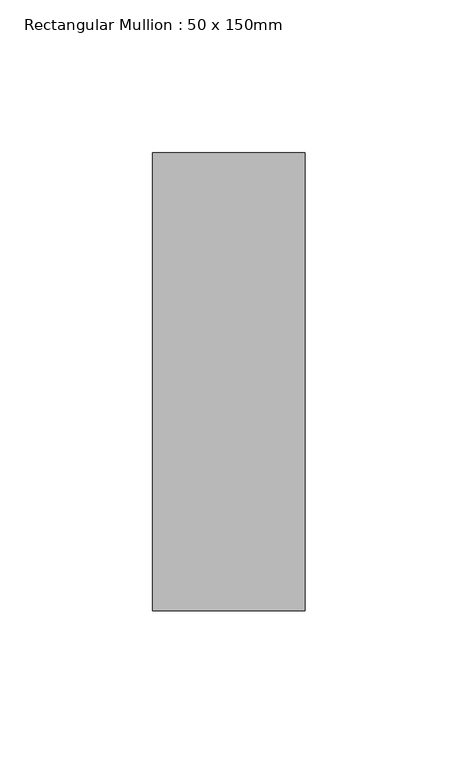
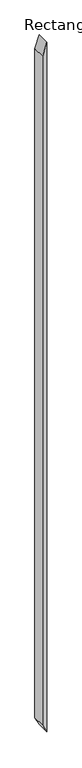
"""IFC4 building model written with IfcOpenShell, lengths in millimetres: member geometry, Rectangular Mullion : 50 x 150mm."""

from ifc_helpers import new_model, si_unit, frame, origin, place, context, project, spatial, polyline, outline, extrude, source, transform, mapped, element, save


def rectangular_mullion_50_x_150mm_9a9dcb3f(model_context):
    return source(origin(), model_context, "Body", "SweptSolid", [
        extrude(outline(polyline([(0.0, 0.0), (-150.2928962, -50.0), (-8210.4264863, -50.0), (-8303.1882256, 0.0), (0.0, 0.0)])), frame((0.0, -75.0, 0.0), z_axis=(0.0, 1.0, 0.0), x_axis=(0.0, 0.0, 1.0)), (0.0, 0.0, 1.0), 150.0),
    ])


if __name__ == "__main__":
    model = new_model("IFC4")
    model_context = context("Model", 3, world=origin())
    ifc_project = project(units=[si_unit("LENGTHUNIT", "METRE", prefix="MILLI")], contexts=[model_context])
    site = spatial("IfcSite", under=ifc_project)
    building = spatial("IfcBuilding", under=site)
    placement = place(None, origin())
    rectangular_mullion_50_x_150mm_shape = rectangular_mullion_50_x_150mm_9a9dcb3f(model_context)
    element("IfcMember", 1, ObjectType="Rectangular Mullion : 50 x 150mm", at=placement, inside=building, context=model_context, shape_type="MappedRepresentation", body=[
        mapped(rectangular_mullion_50_x_150mm_shape, transform((0.0, 0.0, 0.0), x_axis=(1.0, 0.0, 0.0), y_axis=(0.0, 1.0, 0.0), z_axis=(0.0, 0.0, 1.0))),
    ])
    save(model, "model.ifc")

# Revit data of these elements
# Type "Rectangular Mullion : 50 x 150mm"
#   built-in parameter 1007304 = 0.492126 (stored number, unit not read)
#   built-in parameter 1007301 = 0.082021 (stored number, unit not read)
#   built-in parameter 1007300 = 0.082021 (stored number, unit not read)
# Element 1 (IfcMember, "Rectangular Mullion : 50 x 150mm")
#   Materials on its faces: "Metal - Aluminium"
# Materials
#   "Metal - Aluminium": class "Metal", colour RGB 247 247 247, transparency 0
